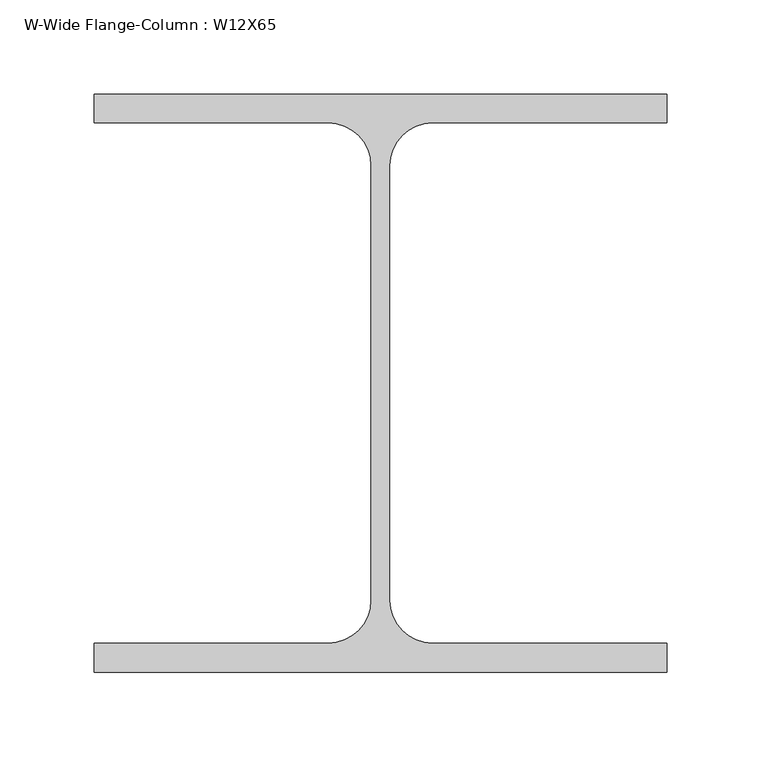
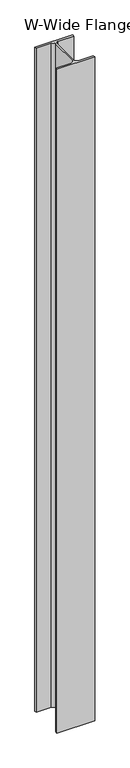
"""IFC4 building model written with IfcOpenShell, lengths in millimetres: column geometry, W-Wide Flange-Column : W12X65."""

from ifc_helpers import new_model, si_unit, point, frame, frame_2d, origin, place, context, project, spatial, polyline, circle_curve, trimmed, segment, composite_curve, outline, extrude, source, transform, mapped, element, save


def w_wide_flange_column_w12x65_95f53b50(model_context):
    return source(origin(), model_context, "Body", "SweptSolid", [
        extrude(outline(composite_curve([segment(polyline([(152.4, 153.67), (152.4, 138.303), (27.686, 138.303)]), True, "CONTINUOUS"), segment(trimmed(circle_curve(frame_2d((27.686, 115.57)), 22.733), [point((27.686, 138.303))], [point((4.953, 115.57))], True, "CARTESIAN"), True, "CONTINUOUS"), segment(polyline([(4.953, 115.57), (4.953, -115.57)]), True, "CONTINUOUS"), segment(trimmed(circle_curve(frame_2d((27.686, -115.57)), 22.733), [point((4.953, -115.57))], [point((27.686, -138.303))], True, "CARTESIAN"), True, "CONTINUOUS"), segment(polyline([(27.686, -138.303), (152.4, -138.303), (152.4, -153.67), (-152.4, -153.67), (-152.4, -138.303), (-27.686, -138.303)]), True, "CONTINUOUS"), segment(trimmed(circle_curve(frame_2d((-27.686, -115.57)), 22.733), [point((-27.686, -138.303))], [point((-4.953, -115.57))], True, "CARTESIAN"), True, "CONTINUOUS"), segment(polyline([(-4.953, -115.57), (-4.953, 115.57)]), True, "CONTINUOUS"), segment(trimmed(circle_curve(frame_2d((-27.686, 115.57)), 22.733), [point((-4.953, 115.57))], [point((-27.686, 138.303))], True, "CARTESIAN"), True, "CONTINUOUS"), segment(polyline([(-27.686, 138.303), (-152.4, 138.303), (-152.4, 153.67), (152.4, 153.67)]), True, "CONTINUOUS")], self_intersect=False)), frame((0.0, 0.0, 11957.05), z_axis=(0.0, 0.0, 1.0), x_axis=(1.0, 0.0, 0.0)), (0.0, 0.0, 1.0), 5670.55),
    ])


if __name__ == "__main__":
    model = new_model("IFC4")
    model_context = context("Model", 3, world=origin())
    ifc_project = project(units=[si_unit("LENGTHUNIT", "METRE", prefix="MILLI")], contexts=[model_context])
    site = spatial("IfcSite", under=ifc_project)
    building = spatial("IfcBuilding", under=site)
    placement = place(None, origin())
    w_wide_flange_column_w12x65_shape = w_wide_flange_column_w12x65_95f53b50(model_context)
    element("IfcColumn", 1, ObjectType="W-Wide Flange-Column : W12X65", at=placement, inside=building, context=model_context, shape_type="MappedRepresentation", body=[
        mapped(w_wide_flange_column_w12x65_shape, transform((0.0, 0.0, 0.0), x_axis=(1.0, 0.0, 0.0), y_axis=(0.0, 1.0, 0.0), z_axis=(0.0, 0.0, 1.0))),
    ])
    save(model, "model.ifc")

# Revit data of these elements
# Type "W-Wide Flange-Column : W12X65"
#   Assembly Code = "B10"
#   W = 65
#   bf = 1' - 0"
#   d = 1' - 0.1"
#   k = 0' - 1 1/2"
#   kr = 0' - 0.895"
#   tf = 0' - 0.605"
#   tw = 0' - 0.39"
#   A = 0.132639 SF
#   Structural Material [instance default] = Steel ASTM A992
# Element 1 (IfcColumn, "W-Wide Flange-Column : W12X65")
#   Materials on its faces: "Steel ASTM A992"
# Materials
#   "Steel ASTM A992": class "Metal", colour RGB 199 199 199, transparency 0, Description = "Structural steel 50ksi", Cost = 0
